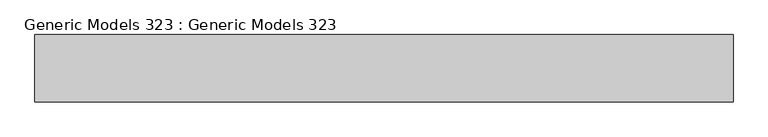
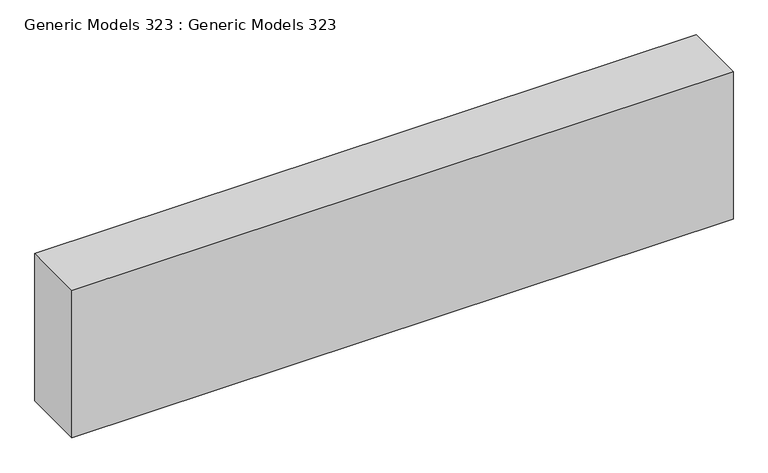
"""IFC4 building model written with IfcOpenShell, lengths in millimetres: proxy geometry, Generic Models 323 : Generic Models 323."""

from ifc_helpers import new_model, si_unit, frame, origin, place, context, project, spatial, polyline, outline, extrude, source, transform, mapped, element, save


def generic_models_323_generic_models_323_0862e19e(model_context):
    return source(origin(), model_context, "Body", "SweptSolid", [
        extrude(outline(polyline([(190.3263704, 1237.9309662), (3339.9263704, 1237.9309662), (3339.9263704, 933.1309662), (190.3263704, 933.1309662), (190.3263704, 1237.9309662)])), frame((0.0, 0.0, 122707.146), z_axis=(0.0, 0.0, 1.0), x_axis=(1.0, 0.0, 0.0)), (0.0, 0.0, 1.0), 742.95),
    ])


if __name__ == "__main__":
    model = new_model("IFC4")
    model_context = context("Model", 3, world=origin())
    ifc_project = project(units=[si_unit("LENGTHUNIT", "METRE", prefix="MILLI")], contexts=[model_context])
    site = spatial("IfcSite", under=ifc_project)
    building = spatial("IfcBuilding", under=site)
    placement = place(None, origin())
    generic_models_323_generic_models_323_shape = generic_models_323_generic_models_323_0862e19e(model_context)
    element("IfcBuildingElementProxy", 1, Name="Generic Models 323 : Generic Models 323", ObjectType="Generic Models 323 : Generic Models 323", at=placement, inside=building, context=model_context, shape_type="MappedRepresentation", body=[
        mapped(generic_models_323_generic_models_323_shape, transform((0.0, 0.0, 0.0), x_axis=(1.0, 0.0, 0.0), y_axis=(0.0, 1.0, 0.0), z_axis=(0.0, 0.0, 1.0))),
    ])
    save(model, "model.ifc")

# Revit data of these elements
# Element 1 (IfcBuildingElementProxy, "Generic Models 323 : Generic Models 323")
#   Materials on its faces: "_CONCRETE SLAB W/ WIRE MESH (SEE STRUCT. DWGS)"
# Materials
#   "_CONCRETE SLAB W/ WIRE MESH (SEE STRUCT. DWGS)": class "Generic", colour RGB 191 191 191, transparency 0, Cost = 0
